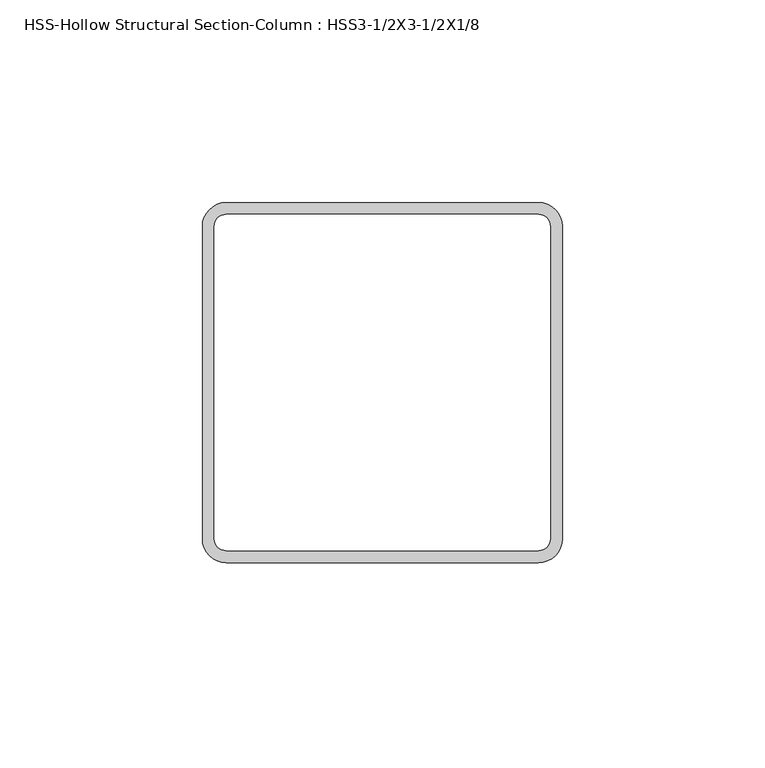
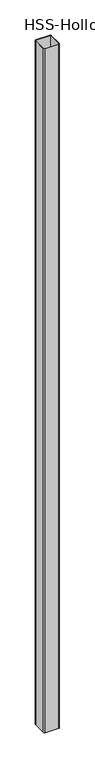
"""IFC4 building model written with IfcOpenShell, lengths in millimetres: column geometry, HSS-Hollow Structural Section-Column : HSS3-1/2X3-1/2X1/8."""

from ifc_helpers import new_model, si_unit, point, frame_2d, origin, origin_with_axes, place, context, project, spatial, polyline, circle_curve, trimmed, segment, composite_curve, outline, extrude, source, transform, mapped, element, save


def hss_hollow_structural_section_column_hss3_1_2x3_1_2x1_8_4949f26d(model_context):
    return source(origin(), model_context, "Body", "SweptSolid", [
        extrude(outline(composite_curve([segment(trimmed(circle_curve(frame_2d((38.5572, 38.5572)), 5.8928), [point((38.5572, 44.45))], [point((44.45, 38.5572))], False, "CARTESIAN"), True, "CONTINUOUS"), segment(polyline([(44.45, 38.5572), (44.45, -38.5572)]), True, "CONTINUOUS"), segment(trimmed(circle_curve(frame_2d((38.5572, -38.5572)), 5.8928), [point((44.45, -38.5572))], [point((38.5572, -44.45))], False, "CARTESIAN"), True, "CONTINUOUS"), segment(polyline([(38.5572, -44.45), (-38.5572, -44.45)]), True, "CONTINUOUS"), segment(trimmed(circle_curve(frame_2d((-38.5572, -38.5572)), 5.8928), [point((-38.5572, -44.45))], [point((-44.45, -38.5572))], False, "CARTESIAN"), True, "CONTINUOUS"), segment(polyline([(-44.45, -38.5572), (-44.45, 38.5572)]), True, "CONTINUOUS"), segment(trimmed(circle_curve(frame_2d((-38.5572, 38.5572)), 5.8928), [point((-44.45, 38.5572))], [point((-38.5572, 44.45))], False, "CARTESIAN"), True, "CONTINUOUS"), segment(polyline([(-38.5572, 44.45), (38.5572, 44.45)]), True, "CONTINUOUS")], self_intersect=False), holes=[composite_curve([segment(polyline([(38.5572, 41.5036), (-38.5572, 41.5036)]), True, "CONTINUOUS"), segment(trimmed(circle_curve(frame_2d((-38.5572, 38.5572)), 2.9464), [point((-38.5572, 41.5036))], [point((-41.5036, 38.5572))], True, "CARTESIAN"), True, "CONTINUOUS"), segment(polyline([(-41.5036, 38.5572), (-41.5036, -38.5572)]), True, "CONTINUOUS"), segment(trimmed(circle_curve(frame_2d((-38.5572, -38.5572)), 2.9464), [point((-41.5036, -38.5572))], [point((-38.5572, -41.5036))], True, "CARTESIAN"), True, "CONTINUOUS"), segment(polyline([(-38.5572, -41.5036), (38.5572, -41.5036)]), True, "CONTINUOUS"), segment(trimmed(circle_curve(frame_2d((38.5572, -38.5572)), 2.9464), [point((38.5572, -41.5036))], [point((41.5036, -38.5572))], True, "CARTESIAN"), True, "CONTINUOUS"), segment(polyline([(41.5036, -38.5572), (41.5036, 38.5572)]), True, "CONTINUOUS"), segment(trimmed(circle_curve(frame_2d((38.5572, 38.5572)), 2.9464), [point((41.5036, 38.5572))], [point((38.5572, 41.5036))], True, "CARTESIAN"), True, "CONTINUOUS")], self_intersect=False)]), origin_with_axes(), (0.0, 0.0, 1.0), 4057.65),
    ])


if __name__ == "__main__":
    model = new_model("IFC4")
    model_context = context("Model", 3, world=origin())
    ifc_project = project(units=[si_unit("LENGTHUNIT", "METRE", prefix="MILLI")], contexts=[model_context])
    site = spatial("IfcSite", under=ifc_project)
    building = spatial("IfcBuilding", under=site)
    placement = place(None, origin())
    hss_hollow_structural_section_column_hss3_1_2x3_1_2x1_8_shape = hss_hollow_structural_section_column_hss3_1_2x3_1_2x1_8_4949f26d(model_context)
    element("IfcColumn", 1, ObjectType="HSS-Hollow Structural Section-Column : HSS3-1/2X3-1/2X1/8", at=placement, inside=building, context=model_context, shape_type="MappedRepresentation", body=[
        mapped(hss_hollow_structural_section_column_hss3_1_2x3_1_2x1_8_shape, transform((0.0, 0.0, 0.0), x_axis=(1.0, 0.0, 0.0), y_axis=(0.0, 1.0, 0.0), z_axis=(0.0, 0.0, 1.0))),
    ])
    save(model, "model.ifc")

# Revit data of these elements
# Type "HSS-Hollow Structural Section-Column : HSS3-1/2X3-1/2X1/8"
#   Keynote = "M05121300.05"
#   Assembly Code = "B10"
#   Shape = "Square"
#   W = 5.6
#   Ht = 0' - 3 1/2"
#   b = 0' - 3 1/2"
#   kr = 0' - 0.232"
#   t = 0' - 0.116"
#   A = 0.0106944 SF
#   Structural Material [instance default] = Steel ASTM A500, Grade B, Rectangular and Square
# Element 1 (IfcColumn, "HSS-Hollow Structural Section-Column : HSS3-1/2X3-1/2X1/8")
#   Materials on its faces: "Steel ASTM A500, Grade B, Rectangular and Square"
# Materials
#   "Steel ASTM A500, Grade B, Rectangular and Square": class "Metal", colour RGB 199 199 199, transparency 0, Description = "Carbon steel", Cost = 0
